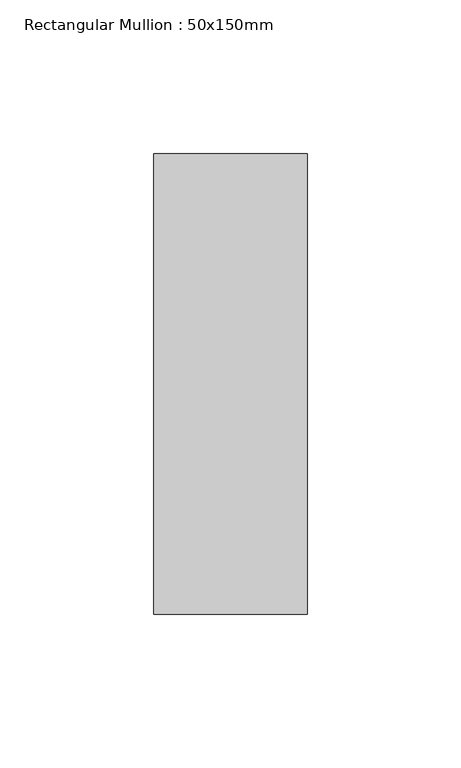
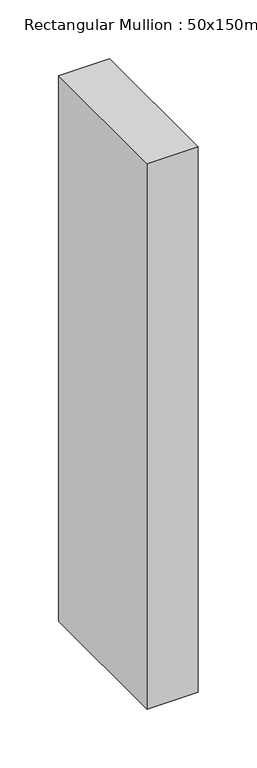
"""IFC4 building model written with IfcOpenShell, lengths in millimetres: member geometry, Rectangular Mullion : 50x150mm."""

from ifc_helpers import new_model, si_unit, frame, origin, place, context, project, spatial, polyline, outline, extrude, source, transform, mapped, element, save


def rectangular_mullion_50x150mm_6f4eac0d(model_context):
    return source(origin(), model_context, "Body", "SweptSolid", [
        extrude(outline(polyline([(0.0, 75.0), (0.0, -75.0), (-50.0, -75.0), (-50.0, 75.0), (0.0, 75.0)])), frame((0.0, 0.0, -564.9999997), z_axis=(0.0, 0.0, 1.0), x_axis=(1.0, 0.0, 0.0)), (0.0, 0.0, 1.0), 564.9999997),
    ])


if __name__ == "__main__":
    model = new_model("IFC4")
    model_context = context("Model", 3, world=origin())
    ifc_project = project(units=[si_unit("LENGTHUNIT", "METRE", prefix="MILLI")], contexts=[model_context])
    site = spatial("IfcSite", under=ifc_project)
    building = spatial("IfcBuilding", under=site)
    placement = place(None, origin())
    rectangular_mullion_50x150mm_shape = rectangular_mullion_50x150mm_6f4eac0d(model_context)
    element("IfcMember", 1, ObjectType="Rectangular Mullion : 50x150mm", at=placement, inside=building, context=model_context, shape_type="MappedRepresentation", body=[
        mapped(rectangular_mullion_50x150mm_shape, transform((0.0, 0.0, 0.0), x_axis=(1.0, 0.0, 0.0), y_axis=(0.0, 1.0, 0.0), z_axis=(0.0, 0.0, 1.0))),
    ])
    save(model, "model.ifc")

# Revit data of these elements
# Type "Rectangular Mullion : 50x150mm"
#   Keynote = "H11"
#   built-in parameter 1007304 = 0.492126 (stored number, unit not read)
#   built-in parameter 1007301 = 0.082021 (stored number, unit not read)
#   built-in parameter 1007300 = 0.082021 (stored number, unit not read)
# Element 1 (IfcMember, "Rectangular Mullion : 50x150mm")
#   Materials on its faces: "Aluminium"
# Materials
#   "Aluminium": class "Metal", colour RGB 247 247 247, transparency 0, Description = "Aluminium 6061", Cost = 0
